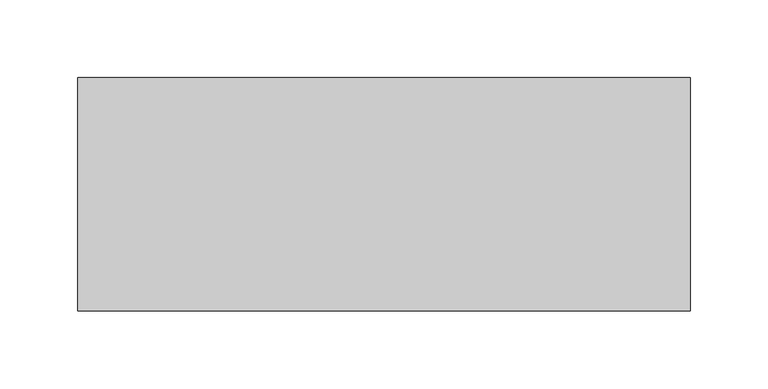
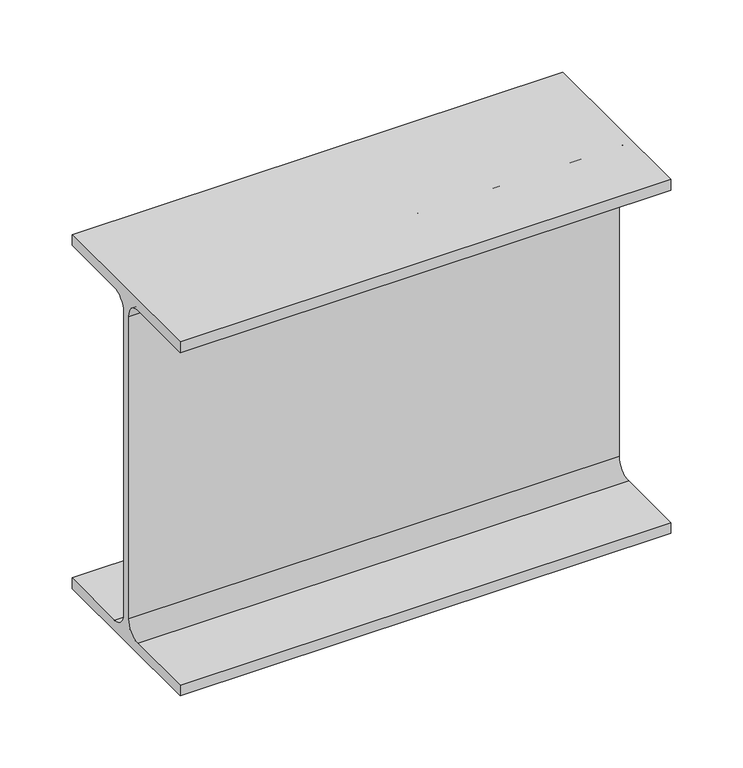
"""IFC4 building model written with IfcOpenShell, lengths in millimetres: beam geometry, 0912_Steel Framing_H-KSD3502 : H_SB_ASB_H-300x150x6.5x9."""

from ifc_helpers import new_model, si_unit, point, frame, frame_2d, origin, place, context, project, spatial, polyline, circle_curve, trimmed, segment, composite_curve, outline, extrude, source, transform, mapped, element, save


def beam_3f731998(model_context):
    return source(origin(), model_context, "Body", "SweptSolid", [
        extrude(outline(composite_curve([segment(polyline([(75.0, -141.0), (75.0, -150.0), (-75.0, -150.0), (-75.0, -141.0), (-16.25, -141.0)]), True, "CONTINUOUS"), segment(trimmed(circle_curve(frame_2d((-16.25, -128.0)), 13.0), [point((-16.25, -141.0))], [point((-3.25, -128.0))], True, "CARTESIAN"), True, "CONTINUOUS"), segment(polyline([(-3.25, -128.0), (-3.25, 128.0)]), True, "CONTINUOUS"), segment(trimmed(circle_curve(frame_2d((-16.25, 128.0)), 13.0), [point((-3.25, 128.0))], [point((-16.25, 141.0))], True, "CARTESIAN"), True, "CONTINUOUS"), segment(polyline([(-16.25, 141.0), (-75.0, 141.0), (-75.0, 150.0), (75.0, 150.0), (75.0, 141.0), (16.25, 141.0)]), True, "CONTINUOUS"), segment(trimmed(circle_curve(frame_2d((16.25, 128.0)), 13.0), [point((16.25, 141.0))], [point((3.25, 128.0))], True, "CARTESIAN"), True, "CONTINUOUS"), segment(polyline([(3.25, 128.0), (3.25, -128.0)]), True, "CONTINUOUS"), segment(trimmed(circle_curve(frame_2d((16.25, -128.0)), 13.0), [point((3.25, -128.0))], [point((16.25, -141.0))], True, "CARTESIAN"), True, "CONTINUOUS"), segment(polyline([(16.25, -141.0), (75.0, -141.0)]), True, "CONTINUOUS")], self_intersect=False)), frame((-190.2999994, 0.0, 0.0), z_axis=(1.0, 0.0, 0.0), x_axis=(0.0, 1.0, 0.0)), (0.0, 0.0, 1.0), 393.2999994),
    ])


if __name__ == "__main__":
    model = new_model("IFC4")
    model_context = context("Model", 3, world=origin())
    ifc_project = project(units=[si_unit("LENGTHUNIT", "METRE", prefix="MILLI")], contexts=[model_context])
    site = spatial("IfcSite", under=ifc_project)
    building = spatial("IfcBuilding", under=site)
    placement = place(None, origin())
    beam_shape = beam_3f731998(model_context)
    element("IfcBeam", 1, ObjectType="0912_Steel Framing_H-KSD3502 : H_SB_ASB_H-300x150x6.5x9", at=placement, inside=building, context=model_context, shape_type="MappedRepresentation", body=[
        mapped(beam_shape, transform((0.0, 0.0, 0.0), x_axis=(1.0, 0.0, 0.0), y_axis=(0.0, 1.0, 0.0), z_axis=(0.0, 0.0, 1.0))),
    ])
    save(model, "model.ifc")

# Revit data of these elements
# Type "0912_Steel Framing_H-KSD3502 : H_SB_ASB_H-300x150x6.5x9"
#   H_WM Code_1 = "S01AA002-00001 | Main Steel Structure Fabrication Work | Shelter/Building | Medium Steel - Standard (90KG/M>Weight≥30KG/M) | Material: (   )"
#   H_WM Code_2 = "S03AA028-00001 | Main Steel Structure Erection Work | Shelter/Building | Medium Steel (90KG/M>Weight≥30KG/M) | Material: (   )"
#   H_WM Code_3 = "S01AA010-00001 | Main Steel Structure Fabrication Work | Shelter/Building | Steel Painting/Coating | for Non-Fireproofed Steel Surface, Surface Preparation, Primer, Second & Final Coat | Material: (   )"
#   H_Q'ty Cal Type Tag = "SB-Q2"
#   Width = 15.0 cm
#   Web Thickness = 0.65 cm
#   Web Fillet = 1.3 cm
#   Warping Constant = 107000.0 cm⁶
#   W = 0
#   Torsional Moment of Inertia = 9.9539 cm⁴
#   Section Area = 46.78 cm²
#   Plastic Modulus weak axis = 105.0 cm³
#   Plastic Modulus strong axis = 542.0 cm³
#   Perimeter = 1.17 m²/m
#   Nominal Weight = 36.70 kgf/m
#   Moment of Inertia weak axis = 508.00 cm⁴
#   Moment of Inertia strong axis = 7210.00 cm⁴
#   Height = 30.0 cm
#   Flange Thickness = 0.9 cm
#   Elastic Modulus weak axis = 67.7 cm³
#   Elastic Modulus strong axis = 481.0 cm³
#   Centroid Vertical = 15.0 cm
#   Centroid Horizontal = 7.5 cm
#   Ix = 72100000
#   Length [instance default] = 1.5240 m
#   Zx = 542000
#   b = 0.1500 m
#   h = 0.3000 m
#   r = 0.0130 m
#   s = 0.0065 m
#   t = 0.0090 m
#   A = 0.004678 m²
#   Structural Material [instance default] = Steel, 45-345
#   Assembly Code = ""
# Element 1 (IfcBeam, "0912_Steel Framing_H-KSD3502 : H_SB_ASB_H-300x150x6.5x9")
#   Structural Material = none
# Materials
#   "Steel, 45-345": class "Metal", colour RGB 189 187 185, transparency 0, Description = "Steel 345 MPa", Cost = 0
